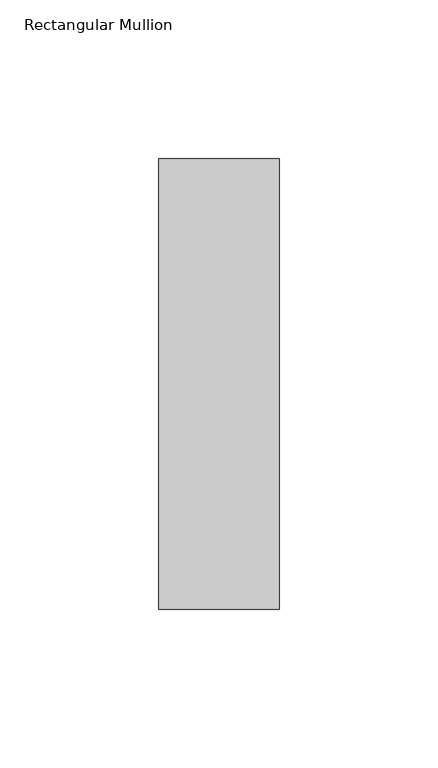
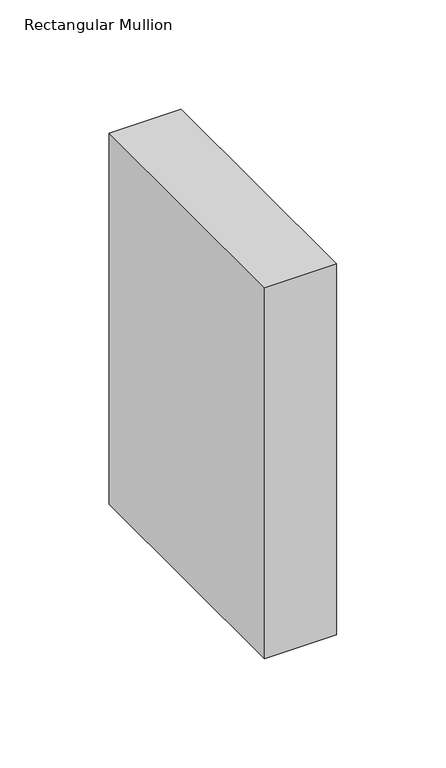
"""IFC4 building model written with IfcOpenShell, lengths in millimetres: member geometry, Rectangular Mullion : NLRS_21_CWM_hsb-regel 38x142_gen_rsf."""

from ifc_helpers import new_model, si_unit, frame, origin, place, context, project, spatial, polyline, outline, extrude, source, transform, mapped, element, save


def rectangular_mullion_345d7182(model_context):
    return source(origin(), model_context, "Body", "SweptSolid", [
        extrude(outline(polyline([(-38.0, -71.0), (-38.0, 71.0), (0.0, 71.0), (0.0, -71.0), (-38.0, -71.0)])), frame((0.0, 0.0, -207.0000003), z_axis=(0.0, 0.0, 1.0), x_axis=(1.0, 0.0, 0.0)), (0.0, 0.0, 1.0), 207.0000003),
    ])


if __name__ == "__main__":
    model = new_model("IFC4")
    model_context = context("Model", 3, world=origin())
    ifc_project = project(units=[si_unit("LENGTHUNIT", "METRE", prefix="MILLI")], contexts=[model_context])
    site = spatial("IfcSite", under=ifc_project)
    building = spatial("IfcBuilding", under=site)
    placement = place(None, origin())
    rectangular_mullion_shape = rectangular_mullion_345d7182(model_context)
    element("IfcMember", 1, ObjectType="Rectangular Mullion : NLRS_21_CWM_hsb-regel 38x142_gen_rsf", at=placement, inside=building, context=model_context, shape_type="MappedRepresentation", body=[
        mapped(rectangular_mullion_shape, transform((0.0, 0.0, 0.0), x_axis=(1.0, 0.0, 0.0), y_axis=(0.0, 1.0, 0.0), z_axis=(0.0, 0.0, 1.0))),
    ])
    save(model, "model.ifc")

# Revit data of these elements
# Type "Rectangular Mullion : NLRS_21_CWM_hsb-regel 38x142_gen_rsf"
#   Export Type to IFC As = "IfcWall"
#   Type IfcGUID = "07M7mRoiH1CR8m_RSKIwpF"
#   Assembly Code = "21.10"
#   built-in parameter 1007322 = 0.465879 (stored number, unit not read)
#   built-in parameter 1007321 = 0.062336 (stored number, unit not read)
#   built-in parameter 1007320 = 0.062336 (stored number, unit not read)
# Element 1 (IfcMember, "Rectangular Mullion : NLRS_21_CWM_hsb-regel 38x142_gen_rsf")
#   Materials on its faces: "NLRS_i2_hout naaldhout vuren_gen_rsf"
# Materials
#   "NLRS_i2_hout naaldhout vuren_gen_rsf": class "I - Hout", colour RGB 234 199 147, transparency 0, Keynote = "i2", Manufacturer = "Revit Standards Foundation", URL = "www.revitstandards.org", Description = "hout vuren", Cost = 0
